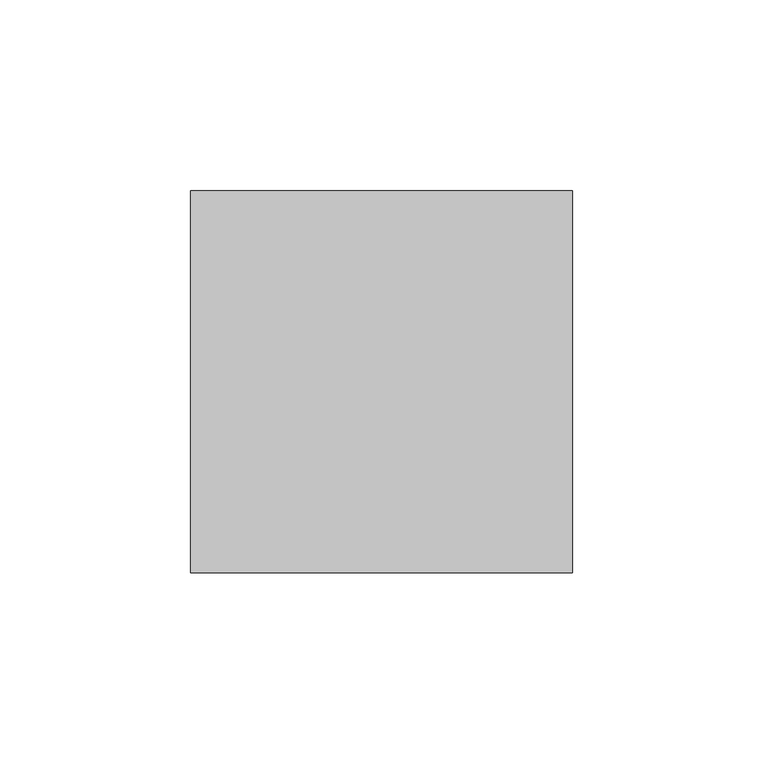
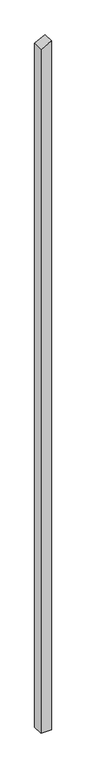
"""IFC4 building model written with IfcOpenShell, lengths in millimetres: column geometry, Holzstütze 159906 : Holzstütze 159906."""

from ifc_helpers import new_model, si_unit, frame, origin, place, context, project, spatial, polyline, outline, extrude, source, transform, mapped, element, save


def column_86400a18(model_context):
    return source(origin(), model_context, "Body", "SweptSolid", [
        extrude(outline(polyline([(-500.0, 157297.7593015), (-500.0, 157397.7593015), (6396.6643707, 157397.7593015), (6345.7118258, 157297.7593015), (-500.0, 157297.7593015)])), frame((0.0, 36959.3988814, 0.0), z_axis=(0.0, 1.0, 0.0), x_axis=(0.0, 0.0, 1.0)), (0.0, 0.0, 1.0), 100.0),
    ])


if __name__ == "__main__":
    model = new_model("IFC4")
    model_context = context("Model", 3, world=origin())
    ifc_project = project(units=[si_unit("LENGTHUNIT", "METRE", prefix="MILLI")], contexts=[model_context])
    site = spatial("IfcSite", under=ifc_project)
    building = spatial("IfcBuilding", under=site)
    placement = place(None, origin())
    column_shape = column_86400a18(model_context)
    element("IfcColumn", 1, ObjectType="Holzstütze 159906 : Holzstütze 159906", at=placement, inside=building, context=model_context, shape_type="MappedRepresentation", body=[
        mapped(column_shape, transform((0.0, 0.0, 0.0), x_axis=(1.0, 0.0, 0.0), y_axis=(0.0, 1.0, 0.0), z_axis=(0.0, 0.0, 1.0))),
    ])
    save(model, "model.ifc")

# Revit data of these elements
# Type "Holzstütze 159906 : Holzstütze 159906"
#   Abrechnungsart = "m"
#   Allright_Bauteil_ID = "0152St 0000143509"
#   Bezeichnung = "Holzstütze"
#   Codetext = "ST-HOLZ\\"
#   Gewerk = "Zimmer- und Holzbauarbeiten"
#   Material = "Holz"
#   Objektname = "Stütze"
#   NameOverride = "Holzstütze"
#   Reference = "Holzstütze"
#   Status = "NEW"
#   ThermalTransmittance = 0.0000 BTU/(h·ft²·°F)
#   Roll = 0.00°
#   Slope = 0.00°
#   2D Interaktion = yes
#   IsExternal = yes
#   LoadBearing = yes
# Element 1 (IfcColumn, "Holzstütze 159906 : Holzstütze 159906")
#   Materials on its faces: "holzschalung"
# Materials
#   "holzschalung": class "Unassigned", colour RGB 128 128 128, transparency 0
